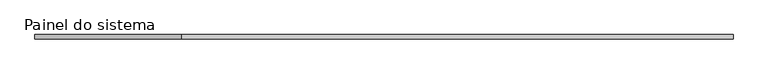
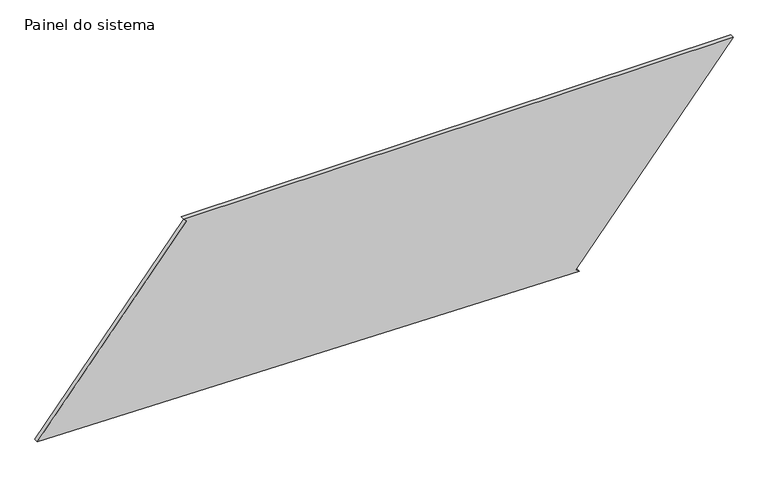
"""IFC4 building model written with IfcOpenShell, lengths in millimetres: plate geometry, Painel do sistema : Envidraçado."""

from ifc_helpers import new_model, si_unit, frame, origin, place, context, project, spatial, polyline, outline, extrude, source, transform, mapped, element, save


def painel_do_sistema_2597e4aa(model_context):
    return source(origin(), model_context, "Body", "SweptSolid", [
        extrude(outline(polyline([(0.0, 1164.4406479), (15.8992441, 1145.1477985), (1162.4295504, 2090.0038358), (1162.4295504, -1211.2567614), (1146.5303063, -1191.9639121), (56.8087527, -2090.0038358), (0.0, 1164.4406479)])), frame((0.0, 24.5, 0.0), z_axis=(0.0, 1.0, 0.0), x_axis=(0.0, 0.0, 1.0)), (0.0, 0.0, 1.0), 25.0),
    ])


if __name__ == "__main__":
    model = new_model("IFC4")
    model_context = context("Model", 3, world=origin())
    ifc_project = project(units=[si_unit("LENGTHUNIT", "METRE", prefix="MILLI")], contexts=[model_context])
    site = spatial("IfcSite", under=ifc_project)
    building = spatial("IfcBuilding", under=site)
    placement = place(None, origin())
    painel_do_sistema_shape = painel_do_sistema_2597e4aa(model_context)
    element("IfcPlate", 1, ObjectType="Painel do sistema : Envidraçado", at=placement, inside=building, context=model_context, shape_type="MappedRepresentation", body=[
        mapped(painel_do_sistema_shape, transform((0.0, 0.0, 0.0), x_axis=(1.0, 0.0, 0.0), y_axis=(0.0, 1.0, 0.0), z_axis=(0.0, 0.0, 1.0))),
    ])
    save(model, "model.ifc")

# Revit data of these elements
# Type "Painel do sistema : Envidraçado"
#   Construction Type Id = "GSP4R"
#   Analytic Construction = "Vidraça única Pilkington 1/8 pol"
#   Visual Light Transmittance = 0.9
#   Solar Heat Gain Coefficient = 0.86
#   Heat Transfer Coefficient (U) = 6.7069 W/(m²·K)
# Element 1 (IfcPlate, "Painel do sistema : Envidraçado")
#   Materials on its faces: "Vidro"
# Materials
#   "Vidro": class "Vidro", colour RGB 0 128 192, transparency 0.9, Description = "Vidro de sílica", Cost = 0
